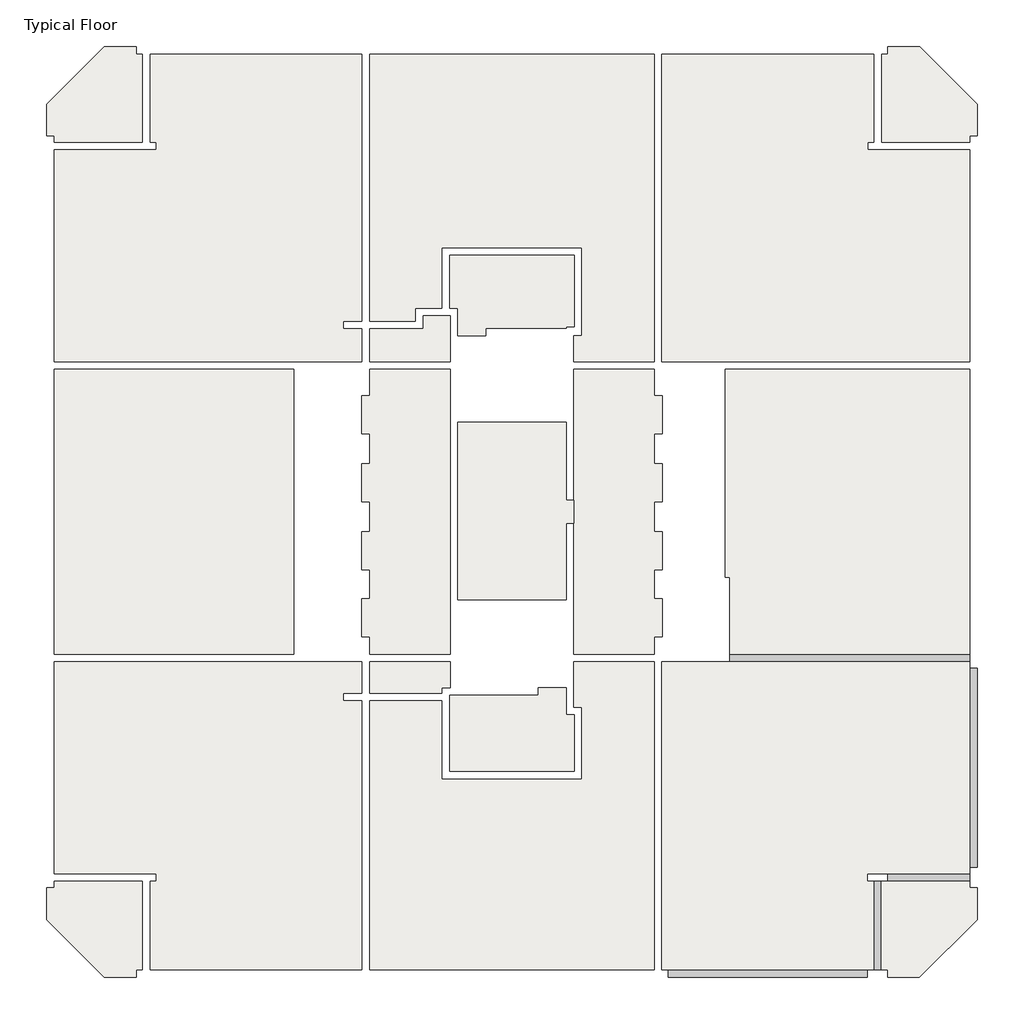
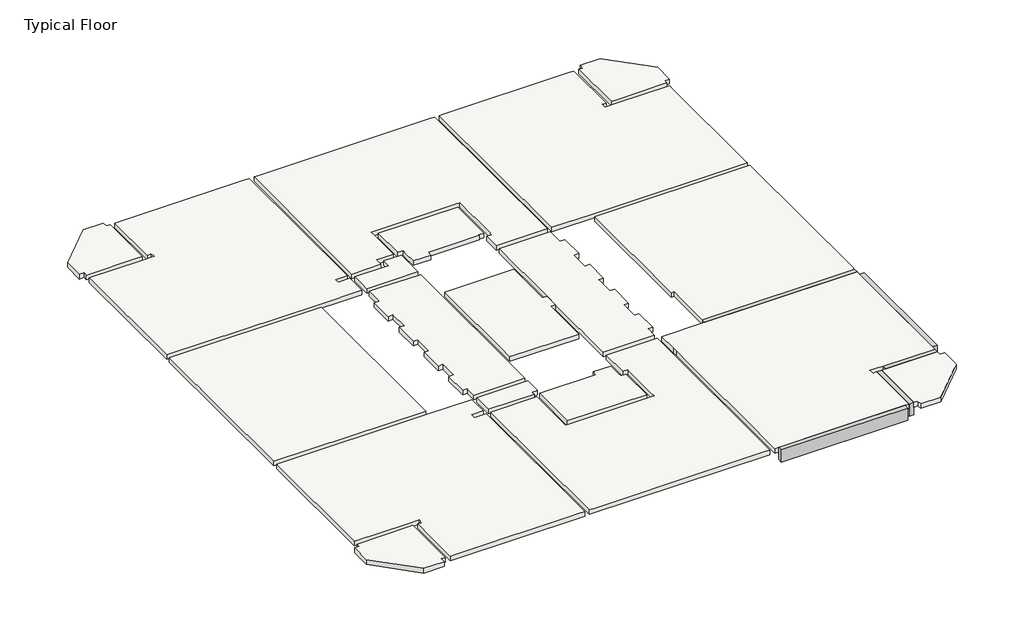
# One storey: 19 slabs, 5 beams.
"""IFC4 building model written with IfcOpenShell, lengths in millimetres."""

import ifcopenshell
import ifcopenshell.guid

model = None  # the IFC model being written
_history = None  # IfcOwnerHistory: only IFC2X3 demands one
_inside = {}  # id of a spatial element -> (the spatial element, [elements in it])
_under = {}  # id of a project, library or spatial element -> (it, [spatial elements below it])
_declared = {}  # id of a project -> (the project, [libraries it declares])
_typed = {}  # id of a type object -> (the type object, [elements of that type])
_made_of = {}  # id of a material, layer set ... -> (it, [elements and type objects made of it])


def new_model(schema):
    """Start an empty IFC model of exactly this schema.

    Asked for "IFC4X3", IfcOpenShell would pick the latest addendum, in which some entities
    have other attributes; the version numbers below select the first issue.
    IFC2X3 requires an IfcOwnerHistory on every rooted entity: one is made here for all.
    """
    global model, _history
    if schema == "IFC4X3":
        model = ifcopenshell.file(schema_version=(4, 3, 0, 0))
    else:
        model = ifcopenshell.file(schema=schema)
    _inside.clear()
    _under.clear()
    _declared.clear()
    _typed.clear()
    _made_of.clear()
    _history = None
    if model.schema == "IFC2X3":
        org = make("IfcOrganization", Name="unknown")
        user = make(
            "IfcPersonAndOrganization",
            ThePerson=make("IfcPerson", FamilyName="unknown"),
            TheOrganization=org,
        )
        app = make(
            "IfcApplication",
            ApplicationDeveloper=org,
            Version="unknown",
            ApplicationFullName="unknown",
            ApplicationIdentifier="unknown",
        )
        _history = make(
            "IfcOwnerHistory",
            OwningUser=user,
            OwningApplication=app,
            ChangeAction="ADDED",
            CreationDate=0,
        )
    return model


def make(cls, **values):
    """One entity of the class cls with the attributes given. An attribute that is None is left unset."""
    return model.create_entity(
        cls, **{name: value for name, value in values.items() if value is not None}
    )


def rooted(cls, **values):
    """An entity with a GlobalId (a new one), such as an element, a storey or a relation."""
    return make(cls, GlobalId=ifcopenshell.guid.new(), OwnerHistory=_history, **values)


def si_unit(unit_type, name, prefix=None):
    """IfcSIUnit, for example si_unit("LENGTHUNIT", "METRE", prefix="MILLI")."""
    return make("IfcSIUnit", UnitType=unit_type, Prefix=prefix, Name=name)


def assignment(units):
    """IfcUnitAssignment: the units of a project."""
    return None if units is None else make("IfcUnitAssignment", Units=units)


def point(xyz):
    """IfcCartesianPoint."""
    return None if xyz is None else make("IfcCartesianPoint", Coordinates=xyz)


def direction(xyz):
    """IfcDirection."""
    return None if xyz is None else make("IfcDirection", DirectionRatios=xyz)


def frame(location, z_axis=None, x_axis=None):
    """IfcAxis2Placement3D, a coordinate frame: its origin and axes. An axis left out is left unset."""
    return make(
        "IfcAxis2Placement3D",
        Location=point(location),
        Axis=direction(z_axis),
        RefDirection=direction(x_axis),
    )


def origin():
    """The frame at (0, 0, 0) with its axes left unset."""
    return frame((0.0, 0.0, 0.0))


def place(relative_to, where):
    """IfcLocalPlacement: puts the frame where relative to a parent placement (None: the world)."""
    return make(
        "IfcLocalPlacement", PlacementRelTo=relative_to, RelativePlacement=where
    )


def context(
    kind, dimensions, precision=None, world=None, true_north=None, identifier=None
):
    """IfcGeometricRepresentationContext, for example the 3D "Model" context."""
    return make(
        "IfcGeometricRepresentationContext",
        ContextIdentifier=identifier,
        ContextType=kind,
        CoordinateSpaceDimension=dimensions,
        Precision=precision,
        WorldCoordinateSystem=world,
        TrueNorth=true_north,
    )


def project(units=None, contexts=None):
    """IfcProject with its units and contexts."""
    return rooted(
        "IfcProject",
        Name="project",
        RepresentationContexts=contexts,
        UnitsInContext=assignment(units),
    )


def spatial(cls, under=None, at=None, **own):
    """A site, building, storey or space (cls), placed at a placement, below another one or the project."""
    s = rooted(cls, ObjectPlacement=at, **own)
    if under is not None:
        _under.setdefault(under.id(), (under, []))[1].append(s)
    return s


def polyline(points):
    """IfcPolyline through the points."""
    return make("IfcPolyline", Points=[point(p) for p in points])


def outline(outer, holes=None, kind="AREA"):
    """IfcArbitraryClosedProfileDef: a profile drawn as a closed curve; with holes, ...WithVoids."""
    if holes is None:
        return make("IfcArbitraryClosedProfileDef", ProfileType=kind, OuterCurve=outer)
    return make(
        "IfcArbitraryProfileDefWithVoids",
        ProfileType=kind,
        OuterCurve=outer,
        InnerCurves=holes,
    )


def extrude(swept, where, along, depth):
    """IfcExtrudedAreaSolid: the profile swept, set in the frame where, extruded along a direction by depth."""
    return make(
        "IfcExtrudedAreaSolid",
        SweptArea=swept,
        Position=where,
        ExtrudedDirection=direction(along),
        Depth=depth,
    )


def faces_of(points, faces, orient=None, outer=None):
    """IfcFace entities. A face is a list of loops; a loop is a list of indices into points, from 0.

    orient and outer hold one flag for each loop. By default every Orientation is true, the
    first loop of a face is its IfcFaceOuterBound and the others are IfcFaceBound.
    """
    made = []
    for i, loops in enumerate(faces):
        bounds = []
        for j, loop in enumerate(loops):
            is_outer = j == 0 if outer is None else outer[i][j]
            bounds.append(
                make(
                    "IfcFaceOuterBound" if is_outer else "IfcFaceBound",
                    Bound=make("IfcPolyLoop", Polygon=[points[k] for k in loop]),
                    Orientation=True if orient is None else orient[i][j],
                )
            )
        made.append(make("IfcFace", Bounds=bounds))
    return made


def faceted_brep(points, faces, orient=None, outer=None, voids=None):
    """IfcFacetedBrep: a solid bounded by flat faces; with voids (closed shells), ...WithVoids."""
    shared = [point(p) for p in points]
    hull = make("IfcClosedShell", CfsFaces=faces_of(shared, faces, orient, outer))
    if voids is None:
        return make("IfcFacetedBrep", Outer=hull)
    return make(
        "IfcFacetedBrepWithVoids",
        Outer=hull,
        Voids=[
            make(cls, CfsFaces=faces_of(shared, fs, o, b)) for cls, fs, o, b in voids
        ],
    )


def shape(context_of_items, identifier, shape_type, items):
    """IfcShapeRepresentation: the items that make up one representation, for example the "Body"."""
    return make(
        "IfcShapeRepresentation",
        ContextOfItems=context_of_items,
        RepresentationIdentifier=identifier,
        RepresentationType=shape_type,
        Items=items,
    )


def made_of(thing, what):
    """Note that an element or type object is made of a material, layer set ...; save() writes the relation."""
    if what is not None:
        _made_of.setdefault(what.id(), (what, []))[1].append(thing)
    return thing


def element(
    cls,
    number,
    at=None,
    inside=None,
    cuts=None,
    type_object=None,
    material=None,
    context=None,
    identifier="Body",
    shape_type=None,
    held_by="IfcProductDefinitionShape",
    body=None,
    shapes=None,
    **own,
):
    """One element of the class cls, such as IfcWall. Its Tag is "e" and its number.

    at: its placement. inside: the storey or other place that contains it. cuts: it is an
    opening in that element (IfcRelVoidsElement). A single representation is given by context,
    identifier, shape_type and body (its items); several are given by shapes. held_by: the class
    of the entity that holds the representations. save() writes the other relations.
    """
    e = rooted(cls, Tag="e%d" % number, ObjectPlacement=at, **own)
    if body is not None:
        shapes = [shape(context, identifier, shape_type, body)]
    if shapes is not None:
        e.Representation = make(held_by, Representations=shapes)
    if inside is not None:
        _inside.setdefault(inside.id(), (inside, []))[1].append(e)
    if cuts is not None:
        rooted(
            "IfcRelVoidsElement", RelatingBuildingElement=cuts, RelatedOpeningElement=e
        )
    if type_object is not None:
        _typed.setdefault(type_object.id(), (type_object, []))[1].append(e)
    return made_of(e, material)


def aggregate(whole, parts):
    """IfcRelAggregates: a whole, such as a stair, and the parts it consists of."""
    return rooted("IfcRelAggregates", RelatingObject=whole, RelatedObjects=parts)


def save(model, path):
    """Write the relations noted so far, then the file.

    IfcRelAggregates (storeys below a building ...), IfcRelContainedInSpatialStructure (elements
    in a storey), IfcRelDefinesByType, IfcRelAssociatesMaterial and IfcRelDeclares: one each for
    every whole, place, type object, material and project.
    """
    for whole, parts in _under.values():
        aggregate(whole, parts)
    for where, things in _inside.values():
        rooted(
            "IfcRelContainedInSpatialStructure",
            RelatedElements=things,
            RelatingStructure=where,
        )
    for kind, things in _typed.values():
        rooted("IfcRelDefinesByType", RelatedObjects=things, RelatingType=kind)
    for what, things in _made_of.values():
        rooted("IfcRelAssociatesMaterial", RelatedObjects=things, RelatingMaterial=what)
    for by, libraries in _declared.values():
        rooted("IfcRelDeclares", RelatingContext=by, RelatedDefinitions=libraries)
    model.write(path)


model = new_model("IFC4")

# Units and contexts
model_context = context("Model", 3, world=origin())
ifc_project = project(units=[si_unit("LENGTHUNIT", "METRE", prefix="MILLI")], contexts=[model_context])

# Site, building, storey
site = spatial("IfcSite", under=ifc_project)
building = spatial("IfcBuilding", under=site)
storey = spatial("IfcBuildingStorey", under=building, Name="Typical Floor", Elevation=3300.0)

# Beams
placement = place(None, origin())
element("IfcBeam", 1, ObjectType="Concrete Rectengular Beam : 30/80", at=placement, inside=storey, context=model_context, shape_type="SweptSolid", body=[
    extrude(outline(polyline([(17474.8160989, -2513.9587131), (17774.8160989, -2513.9587131), (17774.8160989, -10341.2814935), (17474.8160989, -10341.2814935), (17474.8160989, -2513.9587131)])), frame((0.0, 0.0, 2500.0), z_axis=(0.0, 0.0, 1.0), x_axis=(1.0, 0.0, 0.0)), (0.0, 0.0, 1.0), 800.0),
])
element("IfcBeam", 2, ObjectType="Concrete Rectengular Beam : 30/80", at=placement, inside=storey, context=model_context, shape_type="Brep", body=[
    faceted_brep([(14254.5779368, -10591.2814935, 3300.0), (14254.5779368, -10891.2814935, 3300.0), (17474.8160989, -10891.2814935, 3300.0), (17474.8160989, -10591.2814935, 3300.0), (17474.8160989, -10891.2814935, 2500.0), (17474.8160989, -10891.2814935, 3000.0), (14254.5779368, -10891.2814935, 2500.0), (14254.5779368, -10591.2814935, 2500.0), (17474.8160989, -10591.2814935, 2500.0), (17474.8160989, -10591.2814935, 3000.0), (14254.5779368, -10591.2814935, 3000.0)], [[[0, 1, 2, 3]], [[4, 5, 2, 1, 6]], [[6, 7, 8, 4]], [[0, 3, 9, 8, 7, 10]], [[2, 5, 4, 8, 9, 3]], [[1, 0, 10, 7, 6]]]),
])
element("IfcBeam", 3, ObjectType="Concrete Rectengular Beam : 30/80", at=placement, inside=storey, context=model_context, shape_type="Brep", body=[
    faceted_brep([(13704.5779368, -14364.3468097, 3300.0), (14004.5779368, -14364.3468097, 3300.0), (14004.5779368, -10891.2814935, 3300.0), (13704.5779368, -10891.2814935, 3300.0), (13704.5779368, -10891.2814935, 3000.0), (13704.5779368, -10891.2814935, 2500.0), (13704.5779368, -14364.3468097, 2500.0), (13704.5779368, -14364.3468097, 3000.0), (14004.5779368, -14364.3468097, 2500.0), (14004.5779368, -10891.2814935, 2500.0), (14004.5779368, -10891.2814935, 3000.0), (14004.5779368, -14364.3468097, 3000.0)], [[[0, 1, 2, 3]], [[0, 3, 4, 5, 6, 7]], [[8, 6, 5, 9]], [[9, 10, 2, 1, 11, 8]], [[2, 10, 9, 5, 4, 3]], [[1, 0, 7, 6, 8, 11]]]),
])
element("IfcBeam", 4, ObjectType="Concrete Rectengular Beam : 30/80", at=placement, inside=storey, context=model_context, shape_type="SweptSolid", body=[
    extrude(outline(polyline([(13454.5779368, -14364.3468097), (13454.5779368, -14664.3468097), (5623.25294, -14664.3468097), (5623.25294, -14364.3468097), (13454.5779368, -14364.3468097)])), frame((0.0, 0.0, 2500.0), z_axis=(0.0, 0.0, 1.0), x_axis=(1.0, 0.0, 0.0)), (0.0, 0.0, 1.0), 800.0),
])
element("IfcBeam", 5, ObjectType="Concrete Rectengular Beam : 30/80", at=placement, inside=storey, context=model_context, shape_type="Brep", body=[
    faceted_brep([(17474.8160989, -2256.2642878, 3300.0), (17474.8160989, -1956.2642878, 3300.0), (8042.8271106, -1956.2642878, 3300.0), (8042.8271106, -2256.2642878, 3300.0), (17474.8160989, -1956.2642878, 3000.0), (17474.8160989, -1956.2642878, 2500.0), (8042.8271106, -1956.2642878, 2500.0), (8042.8271106, -1956.2642878, 3000.0), (17474.8160989, -2256.2642878, 2500.0), (8042.8271106, -2256.2642878, 2500.0), (17474.8160989, -2256.2642878, 3000.0)], [[[0, 1, 2, 3]], [[1, 4, 5, 6, 7, 2]], [[5, 8, 9, 6]], [[8, 10, 0, 3, 9]], [[0, 10, 8, 5, 4, 1]], [[3, 2, 7, 6, 9]]]),
])

# Slabs
element("IfcSlab", 6, ObjectType="30", at=placement, inside=storey, context=model_context, shape_type="Brep", body=[
    faceted_brep([(-6415.2243211, -2256.2642878, 3000.0), (-6415.2243211, -3492.8093669, 3000.0), (-7145.7620154, -3492.8093669, 3000.0), (-7145.7620154, -3792.8093669, 3000.0), (-6415.2243211, -3792.8093669, 3000.0), (-6415.2243211, -14364.3468097, 3000.0), (-14746.5493178, -14364.3468097, 3000.0), (-14746.5493178, -10891.2814935, 3000.0), (-14496.5493178, -10891.2814935, 3000.0), (-14496.5493178, -10591.2814935, 3000.0), (-15296.5493178, -10591.2814935, 3000.0), (-18516.7874799, -10591.2814935, 3000.0), (-18516.7874799, -2256.2642878, 3000.0), (-6415.2243211, -3492.8093669, 3300.0), (-6415.2243211, -2256.2642878, 3300.0), (-9097.9299438, -2256.2642878, 3300.0), (-18516.7874799, -2256.2642878, 3300.0), (-18516.7874799, -2513.9587131, 3300.0), (-18516.7874799, -10341.2814935, 3300.0), (-18516.7874799, -10591.2814935, 3300.0), (-15296.5493178, -10591.2814935, 3300.0), (-14496.5493178, -10591.2814935, 3300.0), (-14496.5493178, -10891.2814935, 3300.0), (-14746.5493178, -10891.2814935, 3300.0), (-14746.5493178, -14364.3468097, 3300.0), (-14496.5493178, -14364.3468097, 3300.0), (-6665.2243211, -14364.3468097, 3300.0), (-6415.2243211, -14364.3468097, 3300.0), (-6415.2243211, -3792.8093669, 3300.0), (-7145.7620154, -3792.8093669, 3300.0), (-7145.7620154, -3492.8093669, 3300.0)], [[[0, 1, 2, 3, 4, 5, 6, 7, 8, 9, 10, 11, 12]], [[13, 14, 15, 16, 17, 18, 19, 20, 21, 22, 23, 24, 25, 26, 27, 28, 29, 30]], [[1, 0, 14, 13]], [[2, 1, 13, 30]], [[3, 2, 30, 29]], [[4, 3, 29, 28]], [[5, 4, 28, 27]], [[6, 5, 27, 26, 25, 24]], [[7, 6, 24, 23]], [[8, 7, 23, 22]], [[9, 8, 22, 21]], [[9, 21, 20, 19, 11, 10]], [[12, 11, 19, 18, 17, 16]], [[0, 12, 16, 15, 14]]]),
])
element("IfcSlab", 7, ObjectType="30", at=placement, inside=storey, context=model_context, shape_type="Brep", body=[
    faceted_brep([(5373.25294, -3492.8093669, 3000.0), (5373.25294, -2256.2642878, 3000.0), (17474.8160989, -2256.2642878, 3000.0), (17474.8160989, -10591.2814935, 3000.0), (14254.5779368, -10591.2814935, 3000.0), (13454.5779368, -10591.2814935, 3000.0), (13454.5779368, -10891.2814935, 3000.0), (13704.5779368, -10891.2814935, 3000.0), (13704.5779368, -14364.3468097, 3000.0), (5373.25294, -14364.3468097, 3000.0), (5373.25294, -3792.8093669, 3000.0), (5373.25294, -2256.2642878, 3300.0), (5373.25294, -3492.8093669, 3300.0), (5373.25294, -3792.8093669, 3300.0), (5373.25294, -14364.3468097, 3300.0), (5623.25294, -14364.3468097, 3300.0), (13454.5779368, -14364.3468097, 3300.0), (13704.5779368, -14364.3468097, 3300.0), (13704.5779368, -10891.2814935, 3300.0), (13454.5779368, -10891.2814935, 3300.0), (13454.5779368, -10591.2814935, 3300.0), (14254.5779368, -10591.2814935, 3300.0), (17474.8160989, -10591.2814935, 3300.0), (17474.8160989, -10341.2814935, 3300.0), (17474.8160989, -2513.9587131, 3300.0), (17474.8160989, -2256.2642878, 3300.0), (8042.8271106, -2256.2642878, 3300.0)], [[[0, 1, 2, 3, 4, 5, 6, 7, 8, 9, 10]], [[11, 12, 13, 14, 15, 16, 17, 18, 19, 20, 21, 22, 23, 24, 25, 26]], [[1, 0, 12, 11]], [[0, 10, 13, 12]], [[10, 9, 14, 13]], [[9, 8, 17, 16, 15, 14]], [[8, 7, 18, 17]], [[7, 6, 19, 18]], [[6, 5, 20, 19]], [[3, 22, 21, 20, 5, 4]], [[3, 2, 25, 24, 23, 22]], [[2, 1, 11, 26, 25]]]),
])
element("IfcSlab", 8, ObjectType="30", at=placement, inside=storey, context=model_context, shape_type="Brep", body=[
    faceted_brep([(-3270.8136327, -3792.8093669, 3000.0), (-3270.8136327, -6865.8995252, 3000.0), (-2970.8136327, -6865.8995252, 3000.0), (2233.0404623, -6865.8995252, 3000.0), (2233.0404623, -6565.8995252, 3000.0), (2233.0404623, -4336.2642878, 3000.0), (2233.0404623, -4036.2642878, 3000.0), (1915.9035042, -4036.2642878, 3000.0), (1915.9035042, -2256.2642878, 3000.0), (5073.25294, -2256.2642878, 3000.0), (5073.25294, -14364.3468097, 3000.0), (-6115.2243211, -14364.3468097, 3000.0), (-6115.2243211, -3792.8093669, 3000.0), (-3270.8136327, -6865.8995252, 3300.0), (-3270.8136327, -3792.8093669, 3300.0), (-6115.2243211, -3792.8093669, 3300.0), (-6115.2243211, -14364.3468097, 3300.0), (-5865.2243211, -14364.3468097, 3300.0), (4823.25294, -14364.3468097, 3300.0), (5073.25294, -14364.3468097, 3300.0), (5073.25294, -2256.2642878, 3300.0), (4242.4554657, -2256.2642878, 3300.0), (2756.2889137, -2256.2642878, 3300.0), (1915.9035042, -2256.2642878, 3300.0), (1915.9035042, -4036.2642878, 3300.0), (2233.0404623, -4036.2642878, 3300.0), (2233.0404623, -4336.2642878, 3300.0), (2233.0404623, -6565.8995252, 3300.0), (2233.0404623, -6865.8995252, 3300.0), (-2970.8136327, -6865.8995252, 3300.0)], [[[0, 1, 2, 3, 4, 5, 6, 7, 8, 9, 10, 11, 12]], [[13, 14, 15, 16, 17, 18, 19, 20, 21, 22, 23, 24, 25, 26, 27, 28, 29]], [[1, 0, 14, 13]], [[1, 13, 29, 28, 3, 2]], [[3, 28, 27, 26, 25, 6, 5, 4]], [[7, 6, 25, 24]], [[8, 7, 24, 23]], [[9, 8, 23, 22, 21, 20]], [[10, 9, 20, 19]], [[11, 10, 19, 18, 17, 16]], [[12, 11, 16, 15]], [[0, 12, 15, 14]]]),
])
element("IfcSlab", 9, ObjectType="30", at=placement, inside=storey, context=model_context, shape_type="Brep", body=[
    faceted_brep([(13714.5779368, 21634.8017643, 3000.0), (13714.5779368, 18174.5114627, 3000.0), (13464.5779368, 18174.5114627, 3000.0), (13464.5779368, 17874.5114627, 3000.0), (14264.5779368, 17874.5114627, 3000.0), (17474.8160989, 17874.5114627, 3000.0), (17474.8160989, 9551.0309634, 3000.0), (5373.25294, 9551.0309634, 3000.0), (5373.25294, 21634.8017643, 3000.0), (13714.5779368, 18174.5114627, 3300.0), (13714.5779368, 21634.8017643, 3300.0), (13464.5779368, 21634.8017643, 3300.0), (5623.25294, 21634.8017643, 3300.0), (5373.25294, 21634.8017643, 3300.0), (5373.25294, 9551.0309634, 3300.0), (7862.8408752, 9551.0309634, 3300.0), (17474.8160989, 9551.0309634, 3300.0), (17474.8160989, 9786.0412869, 3300.0), (17474.8160989, 17624.5114627, 3300.0), (17474.8160989, 17874.5114627, 3300.0), (14264.5779368, 17874.5114627, 3300.0), (13464.5779368, 17874.5114627, 3300.0), (13464.5779368, 18174.5114627, 3300.0)], [[[0, 1, 2, 3, 4, 5, 6, 7, 8]], [[9, 10, 11, 12, 13, 14, 15, 16, 17, 18, 19, 20, 21, 22]], [[1, 0, 10, 9]], [[2, 1, 9, 22]], [[3, 2, 22, 21]], [[3, 21, 20, 19, 5, 4]], [[6, 5, 19, 18, 17, 16]], [[7, 6, 16, 15, 14]], [[8, 7, 14, 13]], [[0, 8, 13, 12, 11, 10]]]),
])
element("IfcSlab", 10, ObjectType="30", at=placement, inside=storey, context=model_context, shape_type="Brep", body=[
    faceted_brep([(-14746.5493178, 18174.5114627, 3000.0), (-14746.5493178, 21634.8017643, 3000.0), (-6415.2243211, 21634.8017643, 3000.0), (-6415.2243211, 11137.9545698, 3000.0), (-7145.7620154, 11137.9545698, 3000.0), (-7145.7620154, 10837.9545698, 3000.0), (-6415.2243211, 10837.9545698, 3000.0), (-6415.2243211, 9551.0309634, 3000.0), (-18516.7874799, 9551.0309634, 3000.0), (-18516.7874799, 17874.5114627, 3000.0), (-15296.5493178, 17874.5114627, 3000.0), (-14496.5493178, 17874.5114627, 3000.0), (-14496.5493178, 18174.5114627, 3000.0), (-14746.5493178, 21634.8017643, 3300.0), (-14746.5493178, 18174.5114627, 3300.0), (-14496.5493178, 18174.5114627, 3300.0), (-14496.5493178, 17874.5114627, 3300.0), (-15296.5493178, 17874.5114627, 3300.0), (-18516.7874799, 17874.5114627, 3300.0), (-18516.7874799, 17624.5114627, 3300.0), (-18516.7874799, 9786.0412869, 3300.0), (-18516.7874799, 9551.0309634, 3300.0), (-9097.9299438, 9551.0309634, 3300.0), (-6415.2243211, 9551.0309634, 3300.0), (-6415.2243211, 10837.9545698, 3300.0), (-7145.7620154, 10837.9545698, 3300.0), (-7145.7620154, 11137.9545698, 3300.0), (-6415.2243211, 11137.9545698, 3300.0), (-6415.2243211, 21634.8017643, 3300.0), (-6665.2243211, 21634.8017643, 3300.0), (-14496.5493178, 21634.8017643, 3300.0)], [[[0, 1, 2, 3, 4, 5, 6, 7, 8, 9, 10, 11, 12]], [[13, 14, 15, 16, 17, 18, 19, 20, 21, 22, 23, 24, 25, 26, 27, 28, 29, 30]], [[1, 0, 14, 13]], [[0, 12, 15, 14]], [[12, 11, 16, 15]], [[9, 18, 17, 16, 11, 10]], [[9, 8, 21, 20, 19, 18]], [[2, 1, 13, 30, 29, 28]], [[3, 2, 28, 27]], [[4, 3, 27, 26]], [[5, 4, 26, 25]], [[6, 5, 25, 24]], [[7, 6, 24, 23]], [[8, 7, 23, 22, 21]]]),
])
element("IfcSlab", 11, ObjectType="30", at=placement, inside=storey, context=model_context, shape_type="Brep", body=[
    faceted_brep([(-4313.8969087, 11137.9545698, 3000.0), (-6115.2243211, 11137.9545698, 3000.0), (-6115.2243211, 21634.8017643, 3000.0), (5073.25294, 21634.8017643, 3000.0), (5073.25294, 9551.0309634, 3000.0), (1915.9035042, 9551.0309634, 3000.0), (1915.9035042, 10565.0708809, 3000.0), (2233.0404623, 10565.0708809, 3000.0), (2233.0404623, 10915.0708809, 3000.0), (2233.0404623, 14032.7928354, 3000.0), (1933.0404623, 14032.7928354, 3000.0), (-3270.8136327, 14032.7928354, 3000.0), (-3270.8136327, 13732.7928354, 3000.0), (-3270.8136327, 11652.4074259, 3000.0), (-4013.8969087, 11652.4074259, 3000.0), (-4313.8969087, 11652.4074259, 3000.0), (-6115.2243211, 11137.9545698, 3300.0), (-4313.8969087, 11137.9545698, 3300.0), (-4313.8969087, 11652.4074259, 3300.0), (-4013.8969087, 11652.4074259, 3300.0), (-3270.8136327, 11652.4074259, 3300.0), (-3270.8136327, 13732.7928354, 3300.0), (-3270.8136327, 14032.7928354, 3300.0), (1933.0404623, 14032.7928354, 3300.0), (2233.0404623, 14032.7928354, 3300.0), (2233.0404623, 10915.0708809, 3300.0), (2233.0404623, 10565.0708809, 3300.0), (1915.9035042, 10565.0708809, 3300.0), (1915.9035042, 9551.0309634, 3300.0), (2756.2889137, 9551.0309634, 3300.0), (4242.4554657, 9551.0309634, 3300.0), (5073.25294, 9551.0309634, 3300.0), (5073.25294, 21634.8017643, 3300.0), (4823.25294, 21634.8017643, 3300.0), (-5865.2243211, 21634.8017643, 3300.0), (-6115.2243211, 21634.8017643, 3300.0)], [[[0, 1, 2, 3, 4, 5, 6, 7, 8, 9, 10, 11, 12, 13, 14, 15]], [[16, 17, 18, 19, 20, 21, 22, 23, 24, 25, 26, 27, 28, 29, 30, 31, 32, 33, 34, 35]], [[1, 0, 17, 16]], [[2, 1, 16, 35]], [[3, 2, 35, 34, 33, 32]], [[4, 3, 32, 31]], [[5, 4, 31, 30, 29, 28]], [[6, 5, 28, 27]], [[7, 6, 27, 26]], [[7, 26, 25, 24, 9, 8]], [[9, 24, 23, 22, 11, 10]], [[11, 22, 21, 20, 13, 12]], [[13, 20, 19, 18, 15, 14]], [[0, 15, 18, 17]]]),
])
element("IfcSlab", 12, ObjectType="30", at=placement, inside=storey, context=model_context, shape_type="Brep", body=[
    faceted_brep([(17474.8160989, 9251.0309634, 3000.0), (17474.8160989, -1956.2642878, 3000.0), (8042.8271106, -1956.2642878, 3000.0), (8042.8271106, 1064.5202959, 3000.0), (7862.8408752, 1064.5202959, 3000.0), (7862.8408752, 9251.0309634, 3000.0), (17474.8160989, -1956.2642878, 3300.0), (17474.8160989, -1713.9587131, 3300.0), (17474.8160989, 8986.0412869, 3300.0), (17474.8160989, 9251.0309634, 3300.0), (7862.8408752, 9251.0309634, 3300.0), (7862.8408752, 1064.5202959, 3300.0), (8042.8271106, 1064.5202959, 3300.0), (8042.8271106, -1956.2642878, 3300.0)], [[[0, 1, 2, 3, 4, 5]], [[6, 7, 8, 9, 10, 11, 12, 13]], [[1, 0, 9, 8, 7, 6]], [[2, 1, 6, 13]], [[3, 2, 13, 12]], [[4, 3, 12, 11]], [[5, 4, 11, 10]], [[0, 5, 10, 9]]]),
])
element("IfcSlab", 13, ObjectType="30", at=placement, inside=storey, context=model_context, shape_type="Brep", body=[
    faceted_brep([(-9097.9299438, 9251.0309634, 3000.0), (-9097.9299438, -1956.2642878, 3000.0), (-18516.7874799, -1956.2642878, 3000.0), (-18516.7874799, 9251.0309634, 3000.0), (-9097.9299438, 9251.0309634, 3300.0), (-18516.7874799, 9251.0309634, 3300.0), (-18516.7874799, 8986.0412869, 3300.0), (-18516.7874799, -1713.9587131, 3300.0), (-18516.7874799, -1956.2642878, 3300.0), (-9097.9299438, -1956.2642878, 3300.0)], [[[0, 1, 2, 3]], [[4, 5, 6, 7, 8, 9]], [[1, 0, 4, 9]], [[2, 1, 9, 8]], [[3, 2, 8, 7, 6, 5]], [[0, 3, 5, 4]]]),
])
element("IfcSlab", 14, ObjectType="30", at=placement, inside=storey, context=model_context, shape_type="Brep", body=[
    faceted_brep([(-3270.8136327, -3272.2312527, 3000.0), (-3270.8136327, -3492.8093669, 3000.0), (-6115.2243211, -3492.8093669, 3000.0), (-6115.2243211, -2256.2642878, 3000.0), (-5277.5582989, -2256.2642878, 3000.0), (-5277.5582989, -2251.2642878, 3000.0), (-3791.391747, -2251.2642878, 3000.0), (-3791.391747, -2256.2642878, 3000.0), (-2947.5514166, -2256.2642878, 3000.0), (-2947.5514166, -3272.2312527, 3000.0), (-2970.8136327, -3272.2312527, 3000.0), (-3270.8136327, -3492.8093669, 3300.0), (-3270.8136327, -3272.2312527, 3300.0), (-2970.8136327, -3272.2312527, 3300.0), (-2947.5514166, -3272.2312527, 3300.0), (-2947.5514166, -2256.2642878, 3300.0), (-3791.391747, -2256.2642878, 3300.0), (-3791.391747, -2251.2642878, 3300.0), (-5277.5582989, -2251.2642878, 3300.0), (-5277.5582989, -2256.2642878, 3300.0), (-6115.2243211, -2256.2642878, 3300.0), (-6115.2243211, -3492.8093669, 3300.0)], [[[0, 1, 2, 3, 4, 5, 6, 7, 8, 9, 10]], [[11, 12, 13, 14, 15, 16, 17, 18, 19, 20, 21]], [[5, 18, 17, 6]], [[14, 9, 8, 15]], [[9, 14, 13, 12, 0, 10]], [[1, 0, 12, 11]], [[2, 1, 11, 21]], [[2, 21, 20, 3]], [[19, 4, 3, 20]], [[4, 19, 18, 5]], [[7, 16, 15, 8]], [[16, 7, 6, 17]]]),
])
element("IfcSlab", 15, ObjectType="30", at=placement, inside=storey, context=model_context, shape_type="Brep", body=[
    faceted_brep([(-2970.8136327, -3572.2312527, 3000.0), (524.3687486, -3572.2312527, 3000.0), (524.3687486, -3272.2312527, 3000.0), (1615.9035042, -3272.2312527, 3000.0), (1615.9035042, -4036.2642878, 3000.0), (1615.9035042, -4336.2642878, 3000.0), (1933.0404623, -4336.2642878, 3000.0), (1933.0404623, -6565.8995252, 3000.0), (-2970.8136327, -6565.8995252, 3000.0), (524.3687486, -3572.2312527, 3300.0), (-2970.8136327, -3572.2312527, 3300.0), (-2970.8136327, -6565.8995252, 3300.0), (1933.0404623, -6565.8995252, 3300.0), (1933.0404623, -4336.2642878, 3300.0), (1615.9035042, -4336.2642878, 3300.0), (1615.9035042, -4036.2642878, 3300.0), (1615.9035042, -3272.2312527, 3300.0), (524.3687486, -3272.2312527, 3300.0)], [[[0, 1, 2, 3, 4, 5, 6, 7, 8]], [[9, 10, 11, 12, 13, 14, 15, 16, 17]], [[1, 0, 10, 9]], [[2, 1, 9, 17]], [[3, 2, 17, 16]], [[3, 16, 15, 14, 5, 4]], [[6, 5, 14, 13]], [[7, 6, 13, 12]], [[8, 7, 12, 11]], [[0, 8, 11, 10]]]),
])
element("IfcSlab", 16, ObjectType="30", at=placement, inside=storey, context=model_context, shape_type="Brep", body=[
    faceted_brep([(1933.0404623, 13732.7928354, 3000.0), (1933.0404623, 10915.0708809, 3000.0), (1615.9035042, 10915.0708809, 3000.0), (1615.9035042, 10858.9456228, 3000.0), (-1557.9437084, 10858.9456228, 3000.0), (-1557.9437084, 10558.9456228, 3000.0), (-2647.5514166, 10558.9456228, 3000.0), (-2647.5514166, 11352.4074259, 3000.0), (-2647.5514166, 11652.4074259, 3000.0), (-2970.8136327, 11652.4074259, 3000.0), (-2970.8136327, 13732.7928354, 3000.0), (1933.0404623, 10915.0708809, 3300.0), (1933.0404623, 13732.7928354, 3300.0), (-2970.8136327, 13732.7928354, 3300.0), (-2970.8136327, 11652.4074259, 3300.0), (-2647.5514166, 11652.4074259, 3300.0), (-2647.5514166, 11352.4074259, 3300.0), (-2647.5514166, 10558.9456228, 3300.0), (-1557.9437084, 10558.9456228, 3300.0), (-1557.9437084, 10858.9456228, 3300.0), (1615.9035042, 10858.9456228, 3300.0), (1615.9035042, 10915.0708809, 3300.0)], [[[0, 1, 2, 3, 4, 5, 6, 7, 8, 9, 10]], [[11, 12, 13, 14, 15, 16, 17, 18, 19, 20, 21]], [[1, 0, 12, 11]], [[2, 1, 11, 21]], [[3, 2, 21, 20]], [[4, 3, 20, 19]], [[5, 4, 19, 18]], [[6, 5, 18, 17]], [[6, 17, 16, 15, 8, 7]], [[9, 8, 15, 14]], [[10, 9, 14, 13]], [[0, 10, 13, 12]]]),
])
element("IfcSlab", 17, ObjectType="30", at=placement, inside=storey, context=model_context, shape_type="Brep", body=[
    faceted_brep([(-2947.5514166, 9251.0309634, 3000.0), (-2947.5514166, -1956.2642878, 3000.0), (-6119.4715818, -1956.2642878, 3000.0), (-6119.4715818, -1265.4865865, 3000.0), (-6419.4715818, -1265.4865865, 3000.0), (-6419.4715818, 224.8781761, 3000.0), (-6119.4715818, 224.8781761, 3000.0), (-6119.4715818, 1362.5932484, 3000.0), (-6419.4715818, 1362.5932484, 3000.0), (-6419.4715818, 2852.9580109, 3000.0), (-6119.4715818, 2852.9580109, 3000.0), (-6119.4715818, 4041.0516104, 3000.0), (-6419.4715818, 4041.0516104, 3000.0), (-6419.4715818, 5531.4163729, 3000.0), (-6119.4715818, 5531.4163729, 3000.0), (-6119.4715818, 6719.5099724, 3000.0), (-6419.4715818, 6719.5099724, 3000.0), (-6419.4715818, 8205.6765243, 3000.0), (-6119.4715818, 8205.6765243, 3000.0), (-6119.4715818, 9251.0309634, 3000.0), (-2947.5514166, -1956.2642878, 3300.0), (-2947.5514166, 9251.0309634, 3300.0), (-3791.391747, 9251.0309634, 3300.0), (-5277.5582989, 9251.0309634, 3300.0), (-6119.4715818, 9251.0309634, 3300.0), (-6119.4715818, 8205.6765243, 3300.0), (-6419.4715818, 8205.6765243, 3300.0), (-6419.4715818, 6719.5099724, 3300.0), (-6119.4715818, 6719.5099724, 3300.0), (-6119.4715818, 5531.4163729, 3300.0), (-6419.4715818, 5531.4163729, 3300.0), (-6419.4715818, 4041.0516104, 3300.0), (-6119.4715818, 4041.0516104, 3300.0), (-6119.4715818, 2852.9580109, 3300.0), (-6419.4715818, 2852.9580109, 3300.0), (-6419.4715818, 1362.5932484, 3300.0), (-6119.4715818, 1362.5932484, 3300.0), (-6119.4715818, 224.8781761, 3300.0), (-6419.4715818, 224.8781761, 3300.0), (-6419.4715818, -1265.4865865, 3300.0), (-6119.4715818, -1265.4865865, 3300.0), (-6119.4715818, -1956.2642878, 3300.0), (-5277.5582989, -1956.2642878, 3300.0), (-3791.391747, -1956.2642878, 3300.0)], [[[0, 1, 2, 3, 4, 5, 6, 7, 8, 9, 10, 11, 12, 13, 14, 15, 16, 17, 18, 19]], [[20, 21, 22, 23, 24, 25, 26, 27, 28, 29, 30, 31, 32, 33, 34, 35, 36, 37, 38, 39, 40, 41, 42, 43]], [[1, 0, 21, 20]], [[2, 1, 20, 43, 42, 41]], [[0, 19, 24, 23, 22, 21]], [[3, 2, 41, 40]], [[4, 3, 40, 39]], [[5, 4, 39, 38]], [[6, 5, 38, 37]], [[7, 6, 37, 36]], [[8, 7, 36, 35]], [[9, 8, 35, 34]], [[10, 9, 34, 33]], [[11, 10, 33, 32]], [[12, 11, 32, 31]], [[13, 12, 31, 30]], [[14, 13, 30, 29]], [[15, 14, 29, 28]], [[16, 15, 28, 27]], [[17, 16, 27, 26]], [[18, 17, 26, 25]], [[19, 18, 25, 24]]]),
])
element("IfcSlab", 18, ObjectType="30", at=placement, inside=storey, context=model_context, shape_type="Brep", body=[
    faceted_brep([(5084.3687486, -1956.2642878, 3000.0), (1915.9035042, -1956.2642878, 3000.0), (1915.9035042, 3193.7357122, 3000.0), (1915.9035042, 4091.4301376, 3000.0), (1915.9035042, 9251.0309634, 3000.0), (5084.3687486, 9251.0309634, 3000.0), (5084.3687486, 8205.6765243, 3000.0), (5384.3687486, 8205.6765243, 3000.0), (5384.3687486, 6719.5099724, 3000.0), (5084.3687486, 6719.5099724, 3000.0), (5084.3687486, 5531.4163729, 3000.0), (5384.3687486, 5531.4163729, 3000.0), (5384.3687486, 4041.0516104, 3000.0), (5084.3687486, 4041.0516104, 3000.0), (5084.3687486, 2852.9580109, 3000.0), (5384.3687486, 2852.9580109, 3000.0), (5384.3687486, 1362.5932484, 3000.0), (5084.3687486, 1362.5932484, 3000.0), (5084.3687486, 224.8781761, 3000.0), (5384.3687486, 224.8781761, 3000.0), (5384.3687486, -1265.4865865, 3000.0), (5084.3687486, -1265.4865865, 3000.0), (1915.9035042, -1956.2642878, 3300.0), (2756.2889137, -1956.2642878, 3300.0), (4242.4554657, -1956.2642878, 3300.0), (5084.3687486, -1956.2642878, 3300.0), (5084.3687486, -1265.4865865, 3300.0), (5384.3687486, -1265.4865865, 3300.0), (5384.3687486, 224.8781761, 3300.0), (5084.3687486, 224.8781761, 3300.0), (5084.3687486, 1362.5932484, 3300.0), (5384.3687486, 1362.5932484, 3300.0), (5384.3687486, 2852.9580109, 3300.0), (5084.3687486, 2852.9580109, 3300.0), (5084.3687486, 4041.0516104, 3300.0), (5384.3687486, 4041.0516104, 3300.0), (5384.3687486, 5531.4163729, 3300.0), (5084.3687486, 5531.4163729, 3300.0), (5084.3687486, 6719.5099724, 3300.0), (5384.3687486, 6719.5099724, 3300.0), (5384.3687486, 8205.6765243, 3300.0), (5084.3687486, 8205.6765243, 3300.0), (5084.3687486, 9251.0309634, 3300.0), (4242.4554657, 9251.0309634, 3300.0), (2756.2889137, 9251.0309634, 3300.0), (1915.9035042, 9251.0309634, 3300.0), (1915.9035042, 4091.4301376, 3300.0), (1915.9035042, 3193.7357122, 3300.0)], [[[0, 1, 2, 3, 4, 5, 6, 7, 8, 9, 10, 11, 12, 13, 14, 15, 16, 17, 18, 19, 20, 21]], [[22, 23, 24, 25, 26, 27, 28, 29, 30, 31, 32, 33, 34, 35, 36, 37, 38, 39, 40, 41, 42, 43, 44, 45, 46, 47]], [[1, 0, 25, 24, 23, 22]], [[4, 3, 2, 1, 22, 47, 46, 45]], [[5, 4, 45, 44, 43, 42]], [[6, 5, 42, 41]], [[7, 6, 41, 40]], [[8, 7, 40, 39]], [[9, 8, 39, 38]], [[10, 9, 38, 37]], [[11, 10, 37, 36]], [[12, 11, 36, 35]], [[13, 12, 35, 34]], [[14, 13, 34, 33]], [[15, 14, 33, 32]], [[16, 15, 32, 31]], [[17, 16, 31, 30]], [[18, 17, 30, 29]], [[19, 18, 29, 28]], [[20, 19, 28, 27]], [[21, 20, 27, 26]], [[0, 21, 26, 25]]]),
])
element("IfcSlab", 19, ObjectType="30", at=placement, inside=storey, context=model_context, shape_type="SweptSolid", body=[
    extrude(outline(polyline([(1615.9035042, 7164.5202959), (1615.9035042, 4091.4301376), (1915.9035042, 4091.4301376), (1915.9035042, 3193.7357122), (1615.9035042, 3193.7357122), (1615.9035042, 176.4266964), (-2647.5514166, 176.4266964), (-2647.5514166, 7164.5202959), (1615.9035042, 7164.5202959)])), frame((0.0, 0.0, 3000.0), z_axis=(0.0, 0.0, 1.0), x_axis=(1.0, 0.0, 0.0)), (0.0, 0.0, 1.0), 300.0),
])
element("IfcSlab", 20, ObjectType="30", at=placement, inside=storey, context=model_context, shape_type="Brep", body=[
    faceted_brep([(-4013.8969087, 10837.9545698, 3000.0), (-4013.8969087, 11352.4074259, 3000.0), (-2947.5514166, 11352.4074259, 3000.0), (-2947.5514166, 9551.0309634, 3000.0), (-6115.2243211, 9551.0309634, 3000.0), (-6115.2243211, 10837.9545698, 3000.0), (-4313.8969087, 10837.9545698, 3000.0), (-4013.8969087, 11352.4074259, 3300.0), (-4013.8969087, 10837.9545698, 3300.0), (-4313.8969087, 10837.9545698, 3300.0), (-6115.2243211, 10837.9545698, 3300.0), (-6115.2243211, 9551.0309634, 3300.0), (-5277.5582989, 9551.0309634, 3300.0), (-3791.391747, 9551.0309634, 3300.0), (-2947.5514166, 9551.0309634, 3300.0), (-2947.5514166, 11352.4074259, 3300.0)], [[[0, 1, 2, 3, 4, 5, 6]], [[7, 8, 9, 10, 11, 12, 13, 14, 15]], [[8, 0, 6, 5, 10, 9]], [[1, 0, 8, 7]], [[2, 1, 7, 15]], [[3, 2, 15, 14]], [[4, 3, 14, 13, 12, 11]], [[5, 4, 11, 10]]]),
])
element("IfcSlab", 21, ObjectType="30", at=placement, inside=storey, context=model_context, shape_type="Brep", body=[
    faceted_brep([(-18816.7874799, 19669.5636022, 3000.0), (-16551.5493178, 21934.8017643, 3000.0), (-15296.5493178, 21934.8017643, 3000.0), (-15296.5493178, 21634.8017643, 3000.0), (-15046.5493178, 21634.8017643, 3000.0), (-15046.5493178, 18174.5114627, 3000.0), (-18516.7874799, 18174.5114627, 3000.0), (-18516.7874799, 18424.5114627, 3000.0), (-18816.7874799, 18424.5114627, 3000.0), (-16551.5493178, 21934.8017643, 3300.0), (-18816.7874799, 19669.5636022, 3300.0), (-18816.7874799, 18424.5114627, 3300.0), (-18516.7874799, 18424.5114627, 3300.0), (-18516.7874799, 18174.5114627, 3300.0), (-15296.5493178, 18174.5114627, 3300.0), (-15046.5493178, 18174.5114627, 3300.0), (-15046.5493178, 21634.8017643, 3300.0), (-15296.5493178, 21634.8017643, 3300.0), (-15296.5493178, 21934.8017643, 3300.0)], [[[0, 1, 2, 3, 4, 5, 6, 7, 8]], [[9, 10, 11, 12, 13, 14, 15, 16, 17, 18]], [[1, 0, 10, 9]], [[2, 1, 9, 18]], [[3, 2, 18, 17]], [[4, 3, 17, 16]], [[5, 4, 16, 15]], [[6, 5, 15, 14, 13]], [[7, 6, 13, 12]], [[8, 7, 12, 11]], [[0, 8, 11, 10]]]),
])
element("IfcSlab", 22, ObjectType="30", at=placement, inside=storey, context=model_context, shape_type="Brep", body=[
    faceted_brep([(15509.5779368, 21934.8017643, 3000.0), (17774.8160989, 19669.5636022, 3000.0), (17774.8160989, 18424.5114627, 3000.0), (17474.8160989, 18424.5114627, 3000.0), (17474.8160989, 18174.5114627, 3000.0), (14014.5779368, 18174.5114627, 3000.0), (14014.5779368, 21634.8017643, 3000.0), (14264.5779368, 21634.8017643, 3000.0), (14264.5779368, 21934.8017643, 3000.0), (17774.8160989, 19669.5636022, 3300.0), (15509.5779368, 21934.8017643, 3300.0), (14264.5779368, 21934.8017643, 3300.0), (14264.5779368, 21634.8017643, 3300.0), (14014.5779368, 21634.8017643, 3300.0), (14014.5779368, 18174.5114627, 3300.0), (14264.5779368, 18174.5114627, 3300.0), (17474.8160989, 18174.5114627, 3300.0), (17474.8160989, 18424.5114627, 3300.0), (17774.8160989, 18424.5114627, 3300.0)], [[[0, 1, 2, 3, 4, 5, 6, 7, 8]], [[9, 10, 11, 12, 13, 14, 15, 16, 17, 18]], [[1, 0, 10, 9]], [[0, 8, 11, 10]], [[8, 7, 12, 11]], [[7, 6, 13, 12]], [[6, 5, 14, 13]], [[5, 4, 16, 15, 14]], [[4, 3, 17, 16]], [[3, 2, 18, 17]], [[2, 1, 9, 18]]]),
])
element("IfcSlab", 23, ObjectType="30", at=placement, inside=storey, context=model_context, shape_type="Brep", body=[
    faceted_brep([(-16551.5493178, -14664.3468097, 3000.0), (-18816.7874799, -12399.1086476, 3000.0), (-18816.7874799, -11141.2814935, 3000.0), (-18516.7874799, -11141.2814935, 3000.0), (-18516.7874799, -10891.2814935, 3000.0), (-15046.5493178, -10891.2814935, 3000.0), (-15046.5493178, -14364.3468097, 3000.0), (-15296.5493178, -14364.3468097, 3000.0), (-15296.5493178, -14664.3468097, 3000.0), (-18816.7874799, -12399.1086476, 3300.0), (-16551.5493178, -14664.3468097, 3300.0), (-15296.5493178, -14664.3468097, 3300.0), (-15296.5493178, -14364.3468097, 3300.0), (-15046.5493178, -14364.3468097, 3300.0), (-15046.5493178, -10891.2814935, 3300.0), (-15296.5493178, -10891.2814935, 3300.0), (-18516.7874799, -10891.2814935, 3300.0), (-18516.7874799, -11141.2814935, 3300.0), (-18816.7874799, -11141.2814935, 3300.0)], [[[0, 1, 2, 3, 4, 5, 6, 7, 8]], [[9, 10, 11, 12, 13, 14, 15, 16, 17, 18]], [[1, 0, 10, 9]], [[0, 8, 11, 10]], [[8, 7, 12, 11]], [[7, 6, 13, 12]], [[6, 5, 14, 13]], [[5, 4, 16, 15, 14]], [[4, 3, 17, 16]], [[3, 2, 18, 17]], [[2, 1, 9, 18]]]),
])
element("IfcSlab", 24, ObjectType="30", at=placement, inside=storey, context=model_context, shape_type="Brep", body=[
    faceted_brep([(17774.8160989, -12386.333633, 3000.0), (15496.8029222, -14664.3468097, 3000.0), (14254.5779368, -14664.3468097, 3000.0), (14254.5779368, -14364.3468097, 3000.0), (14004.5779368, -14364.3468097, 3000.0), (14004.5779368, -10891.2814935, 3000.0), (17474.8160989, -10891.2814935, 3000.0), (17474.8160989, -11141.2814935, 3000.0), (17774.8160989, -11141.2814935, 3000.0), (15496.8029222, -14664.3468097, 3300.0), (17774.8160989, -12386.333633, 3300.0), (17774.8160989, -11141.2814935, 3300.0), (17474.8160989, -11141.2814935, 3300.0), (17474.8160989, -10891.2814935, 3300.0), (14254.5779368, -10891.2814935, 3300.0), (14004.5779368, -10891.2814935, 3300.0), (14004.5779368, -14364.3468097, 3300.0), (14254.5779368, -14364.3468097, 3300.0), (14254.5779368, -14664.3468097, 3300.0)], [[[0, 1, 2, 3, 4, 5, 6, 7, 8]], [[9, 10, 11, 12, 13, 14, 15, 16, 17, 18]], [[1, 0, 10, 9]], [[2, 1, 9, 18]], [[3, 2, 18, 17]], [[4, 3, 17, 16]], [[5, 4, 16, 15]], [[6, 5, 15, 14, 13]], [[7, 6, 13, 12]], [[8, 7, 12, 11]], [[0, 8, 11, 10]]]),
])

save(model, "model.ifc")

# Revit data of these elements
# Type "Concrete Rectengular Beam : 30/80"
#   Length [instance default] = 152.4 cm
#   b = 30 cm
#   h = 80 cm
#   Structural Material [instance default] = Concrete
#   Assembly Code = ""
# Type "30"
#   Function = 0
#   Layers, outside or top first: 30 cm "Concrete" (function 1)
# Element 1 (IfcBeam, "Concrete Rectengular Beam : 30/80")
#   Comments = ""
#   Mark = "B6"
#   SOFiSTiK_AMG_Comments = ""
#   SOFiSTiK_AMG_Scheduled = yes
#   SOFiSTiK_AMG_Adjusted = yes
#   Structural Material = Concrete
#   Phase Created = New Construction
#   Materials on its faces: "Concrete"
# Element 2 (IfcBeam, "Concrete Rectengular Beam : 30/80")
#   Comments = ""
#   Mark = "B7"
#   SOFiSTiK_AMG_Comments = ""
#   SOFiSTiK_AMG_Scheduled = yes
#   SOFiSTiK_AMG_Adjusted = yes
#   Structural Material = Concrete
#   Phase Created = New Construction
#   Materials on its faces: "Concrete"
# Element 3 (IfcBeam, "Concrete Rectengular Beam : 30/80")
#   Comments = ""
#   Mark = "B8"
#   SOFiSTiK_AMG_Comments = ""
#   SOFiSTiK_AMG_Scheduled = yes
#   SOFiSTiK_AMG_Adjusted = yes
#   Structural Material = Concrete
#   Phase Created = New Construction
#   Materials on its faces: "Concrete"
# Element 4 (IfcBeam, "Concrete Rectengular Beam : 30/80")
#   Comments = ""
#   Mark = "B9"
#   SOFiSTiK_AMG_Comments = ""
#   SOFiSTiK_AMG_Scheduled = yes
#   SOFiSTiK_AMG_Adjusted = yes
#   Structural Material = Concrete
#   Phase Created = New Construction
#   Materials on its faces: "Concrete"
# Element 5 (IfcBeam, "Concrete Rectengular Beam : 30/80")
#   Comments = ""
#   Mark = "B10"
#   SOFiSTiK_AMG_Comments = ""
#   SOFiSTiK_AMG_Scheduled = yes
#   SOFiSTiK_AMG_Adjusted = yes
#   Structural Material = Concrete
#   Phase Created = New Construction
#   Materials on its faces: "Concrete"
# Element 6 (IfcSlab, "30")
#   Mark = "S1"
#   SOFiSTiK_AMG_Comments = ""
#   Height Offset From Level = 0 cm
#   built-in parameter 1001954 = 1
#   SOFiSTiK_AMG_Scheduled = yes
#   SOFiSTiK_AMG_Adjusted = no
#   Phase Created = New Construction
#   Materials on its faces: "Concrete"
# Element 7 (IfcSlab, "30")
#   Mark = "S2"
#   SOFiSTiK_AMG_Comments = ""
#   built-in parameter 1001955 = 3.14159 (stored number, unit not read)
#   Height Offset From Level = 0 cm
#   built-in parameter 1001954 = 1
#   SOFiSTiK_AMG_Scheduled = yes
#   SOFiSTiK_AMG_Adjusted = no
#   Phase Created = New Construction
#   Materials on its faces: "Concrete"
# Element 8 (IfcSlab, "30")
#   Mark = "S3"
#   SOFiSTiK_AMG_Comments = ""
#   Height Offset From Level = 0 cm
#   built-in parameter 1001954 = 1
#   SOFiSTiK_AMG_Scheduled = yes
#   SOFiSTiK_AMG_Adjusted = yes
#   Phase Created = New Construction
#   Materials on its faces: "Concrete"
# Element 9 (IfcSlab, "30")
#   Mark = "S4"
#   SOFiSTiK_AMG_Comments = ""
#   Height Offset From Level = 0 cm
#   built-in parameter 1001954 = 1
#   SOFiSTiK_AMG_Scheduled = yes
#   SOFiSTiK_AMG_Adjusted = no
#   Phase Created = New Construction
#   Materials on its faces: "Concrete"
# Element 10 (IfcSlab, "30")
#   Mark = "S5"
#   SOFiSTiK_AMG_Comments = ""
#   built-in parameter 1001955 = 3.14159 (stored number, unit not read)
#   Height Offset From Level = 0 cm
#   built-in parameter 1001954 = 1
#   SOFiSTiK_AMG_Scheduled = yes
#   SOFiSTiK_AMG_Adjusted = no
#   Phase Created = New Construction
#   Materials on its faces: "Concrete"
# Element 11 (IfcSlab, "30")
#   Mark = "S6"
#   SOFiSTiK_AMG_Comments = ""
#   Height Offset From Level = 0 cm
#   built-in parameter 1001954 = 1
#   SOFiSTiK_AMG_Scheduled = yes
#   SOFiSTiK_AMG_Adjusted = yes
#   Phase Created = New Construction
#   Materials on its faces: "Concrete"
# Element 12 (IfcSlab, "30")
#   Mark = "S7"
#   SOFiSTiK_AMG_Comments = ""
#   Height Offset From Level = 0 cm
#   built-in parameter 1001954 = 1
#   SOFiSTiK_AMG_Scheduled = yes
#   SOFiSTiK_AMG_Adjusted = yes
#   Phase Created = New Construction
#   Materials on its faces: "Concrete"
# Element 13 (IfcSlab, "30")
#   Mark = "S8"
#   SOFiSTiK_AMG_Comments = ""
#   Height Offset From Level = 0 cm
#   built-in parameter 1001954 = 1
#   SOFiSTiK_AMG_Scheduled = yes
#   SOFiSTiK_AMG_Adjusted = yes
#   Phase Created = New Construction
#   Materials on its faces: "Concrete"
# Element 14 (IfcSlab, "30")
#   Mark = "S9"
#   SOFiSTiK_AMG_Comments = ""
#   built-in parameter 1001955 = 1.5708 (stored number, unit not read)
#   Height Offset From Level = 0 cm
#   built-in parameter 1001954 = 1
#   SOFiSTiK_AMG_Scheduled = yes
#   SOFiSTiK_AMG_Adjusted = yes
#   Phase Created = New Construction
#   Materials on its faces: "Concrete"
# Element 15 (IfcSlab, "30")
#   Mark = "S10"
#   SOFiSTiK_AMG_Comments = ""
#   built-in parameter 1001955 = 1.5708 (stored number, unit not read)
#   Height Offset From Level = 0 cm
#   built-in parameter 1001954 = 1
#   SOFiSTiK_AMG_Scheduled = yes
#   SOFiSTiK_AMG_Adjusted = yes
#   Phase Created = New Construction
#   Materials on its faces: "Concrete"
# Element 16 (IfcSlab, "30")
#   Mark = "S11"
#   SOFiSTiK_AMG_Comments = ""
#   Height Offset From Level = 0 cm
#   built-in parameter 1001954 = 1
#   SOFiSTiK_AMG_Scheduled = yes
#   SOFiSTiK_AMG_Adjusted = yes
#   Phase Created = New Construction
#   Materials on its faces: "Concrete"
# Element 17 (IfcSlab, "30")
#   Mark = "S12"
#   SOFiSTiK_AMG_Comments = ""
#   Height Offset From Level = 0 cm
#   built-in parameter 1001954 = 1
#   SOFiSTiK_AMG_Scheduled = yes
#   SOFiSTiK_AMG_Adjusted = yes
#   Phase Created = New Construction
#   Materials on its faces: "Concrete"
# Element 18 (IfcSlab, "30")
#   Mark = "S13"
#   SOFiSTiK_AMG_Comments = ""
#   Height Offset From Level = 0 cm
#   built-in parameter 1001954 = 1
#   SOFiSTiK_AMG_Scheduled = yes
#   SOFiSTiK_AMG_Adjusted = yes
#   Phase Created = New Construction
#   Materials on its faces: "Concrete"
# Element 19 (IfcSlab, "30")
#   Mark = "S14"
#   SOFiSTiK_AMG_Comments = ""
#   Height Offset From Level = 0 cm
#   built-in parameter 1001954 = 1
#   SOFiSTiK_AMG_Scheduled = yes
#   SOFiSTiK_AMG_Adjusted = yes
#   Phase Created = New Construction
#   Materials on its faces: "Concrete"
# Element 20 (IfcSlab, "30")
#   Mark = "S15"
#   SOFiSTiK_AMG_Comments = ""
#   built-in parameter 1001955 = 1.5708 (stored number, unit not read)
#   Height Offset From Level = 0 cm
#   built-in parameter 1001954 = 1
#   SOFiSTiK_AMG_Scheduled = yes
#   SOFiSTiK_AMG_Adjusted = yes
#   Phase Created = New Construction
#   Materials on its faces: "Concrete"
# Element 21 (IfcSlab, "30")
#   Mark = "S16"
#   SOFiSTiK_AMG_Comments = ""
#   built-in parameter 1001955 = 3.14159 (stored number, unit not read)
#   Height Offset From Level = 0 cm
#   built-in parameter 1001954 = 1
#   SOFiSTiK_AMG_Scheduled = yes
#   SOFiSTiK_AMG_Adjusted = yes
#   Phase Created = New Construction
#   Materials on its faces: "Concrete"
# Element 22 (IfcSlab, "30")
#   Mark = "S17"
#   SOFiSTiK_AMG_Comments = ""
#   built-in parameter 1001955 = 0 (stored number, unit not read)
#   Height Offset From Level = 0 cm
#   built-in parameter 1001954 = 1
#   SOFiSTiK_AMG_Scheduled = yes
#   SOFiSTiK_AMG_Adjusted = yes
#   Phase Created = New Construction
#   Materials on its faces: "Concrete"
# Element 23 (IfcSlab, "30")
#   Mark = "S18"
#   SOFiSTiK_AMG_Comments = ""
#   built-in parameter 1001955 = 3.14159 (stored number, unit not read)
#   Height Offset From Level = 0 cm
#   built-in parameter 1001954 = 1
#   SOFiSTiK_AMG_Scheduled = yes
#   SOFiSTiK_AMG_Adjusted = yes
#   Phase Created = New Construction
#   Materials on its faces: "Concrete"
# Element 24 (IfcSlab, "30")
#   Mark = "S19"
#   SOFiSTiK_AMG_Comments = ""
#   built-in parameter 1001955 = 0 (stored number, unit not read)
#   Height Offset From Level = 0 cm
#   built-in parameter 1001954 = 1
#   SOFiSTiK_AMG_Scheduled = yes
#   SOFiSTiK_AMG_Adjusted = yes
#   Phase Created = New Construction
#   Materials on its faces: "Concrete"
# Materials
#   "Concrete": class "Concrete", colour RGB 192 192 192, transparency 0, Keynote = "01000", Description = "Cast-in-place concrete", Cost = 0
